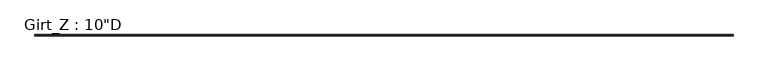
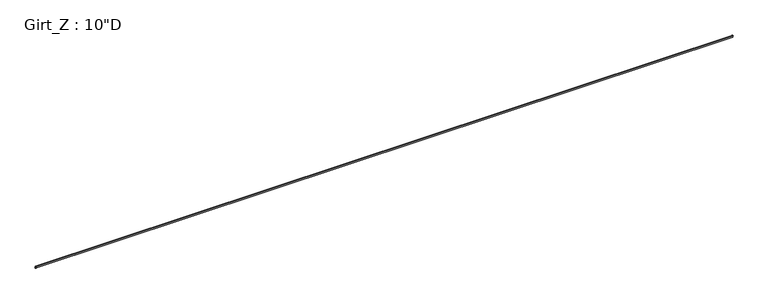
"""IFC4 building model written with IfcOpenShell, lengths in millimetres: beam geometry."""

from ifc_helpers import new_model, si_unit, point, frame, frame_2d, origin, place, context, project, spatial, polyline, circle_curve, trimmed, segment, composite_curve, outline, extrude, source, transform, mapped, element, save


def beam_d420888b(model_context):
    return source(origin(), model_context, "Body", "SweptSolid", [
        extrude(outline(composite_curve([segment(polyline([(-77.9859375, 127.0), (-3.3734375, 127.0)]), True, "CONTINUOUS"), segment(trimmed(circle_curve(frame_2d((-3.3734375, 122.2375)), 4.7625), [point((-3.3734375, 127.0))], [point((1.3890625, 122.2375))], False, "CARTESIAN"), True, "CONTINUOUS"), segment(polyline([(1.3890625, 122.2375), (1.3890625, -122.2389339)]), True, "CONTINUOUS"), segment(trimmed(circle_curve(frame_2d((3.3748024, -122.2389339)), 1.9857399), [point((1.3890625, -122.2389339))], [point((3.2694106, -124.221875))], True, "CARTESIAN"), True, "CONTINUOUS"), segment(polyline([(3.2694106, -124.221875), (83.0404765, -124.221875), (94.4528742, -110.621109), (96.5810415, -112.4068534), (84.3359375, -127.0), (-1.3890625, -127.0), (-1.3890625, 122.2381931)]), True, "CONTINUOUS"), segment(trimmed(circle_curve(frame_2d((-3.3741066, 122.2381931)), 1.9850441), [point((-1.3890625, 122.2381931))], [point((-3.3005807, 124.221875))], True, "CARTESIAN"), True, "CONTINUOUS"), segment(polyline([(-3.3005807, 124.221875), (-76.6904765, 124.221875), (-88.1028742, 110.621109), (-90.2310415, 112.4068534), (-77.9859375, 127.0)]), True, "CONTINUOUS")], self_intersect=False)), frame((-41099.994, 0.0, 0.0), z_axis=(1.0, 0.0, 0.0), x_axis=(0.0, 1.0, 0.0)), (0.0, 0.0, 1.0), 82222.594),
    ])


if __name__ == "__main__":
    model = new_model("IFC4")
    model_context = context("Model", 3, world=origin())
    ifc_project = project(units=[si_unit("LENGTHUNIT", "METRE", prefix="MILLI")], contexts=[model_context])
    site = spatial("IfcSite", under=ifc_project)
    building = spatial("IfcBuilding", under=site)
    placement = place(None, origin())
    beam_shape = beam_d420888b(model_context)
    element("IfcBeam", 1, ObjectType="Girt_Z : 10\"D", at=placement, inside=building, context=model_context, shape_type="MappedRepresentation", body=[
        mapped(beam_shape, transform((0.0, 0.0, 0.0), x_axis=(1.0, 0.0, 0.0), y_axis=(0.0, 1.0, 0.0), z_axis=(0.0, 0.0, 1.0))),
    ])
    save(model, "model.ifc")

# Revit data of these elements
# Type "Girt_Z : 10\"D"
#   half leg = 0' - 1 11/16"
#   Web_Thickness = 0' - 0 7/64"
#   Length [instance default] = 10' - 0"
#   Leg_2 = 0' - 3 3/8"
#   Leg_1 = 0' - 3 1/8"
#   Height = 0' - 10"
#   Structural Material [instance default] = none
